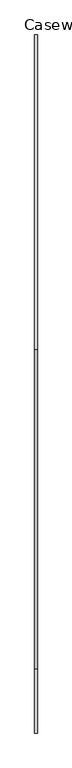
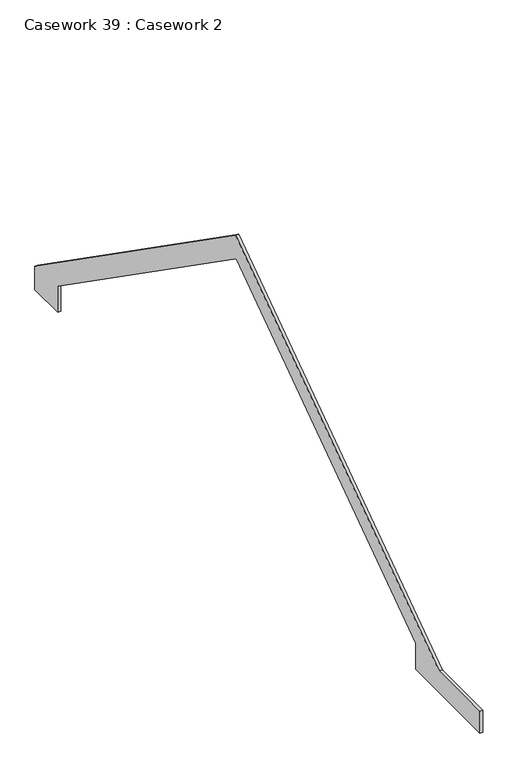
"""IFC4 building model written with IfcOpenShell, lengths in millimetres: furniture geometry, Casework 39 : Casework 2."""

from ifc_helpers import new_model, si_unit, frame, origin, place, context, project, spatial, polyline, outline, extrude, source, transform, mapped, element, save


def casework_39_casework_2_646cf92f(model_context):
    return source(origin(), model_context, "Body", "SweptSolid", [
        extrude(outline(polyline([(3156.9704867, 7937.1283557), (7125.8166964, 5158.1123216), (7125.8166964, 4875.3461918), (6675.8166964, 4875.3461918), (6675.8166964, 5190.0895255), (3151.1408768, 7658.0941041), (-400.040882, 5171.5298671), (-400.040882, 4860.0), (-1669.6462381, 4860.0), (-1669.6462381, 5121.8983063), (-863.5946969, 5121.8983063), (3156.9704867, 7937.1283557)])), frame((713.8336886, 0.0, 0.0), z_axis=(1.0, 0.0, 0.0), x_axis=(0.0, 1.0, 0.0)), (0.0, 0.0, 1.0), 33.2089356),
    ])


if __name__ == "__main__":
    model = new_model("IFC4")
    model_context = context("Model", 3, world=origin())
    ifc_project = project(units=[si_unit("LENGTHUNIT", "METRE", prefix="MILLI")], contexts=[model_context])
    site = spatial("IfcSite", under=ifc_project)
    building = spatial("IfcBuilding", under=site)
    placement = place(None, origin())
    casework_39_casework_2_shape = casework_39_casework_2_646cf92f(model_context)
    element("IfcFurniture", 1, ObjectType="Casework 39 : Casework 2", at=placement, inside=building, context=model_context, shape_type="MappedRepresentation", body=[
        mapped(casework_39_casework_2_shape, transform((0.0, 0.0, 0.0), x_axis=(1.0, 0.0, 0.0), y_axis=(0.0, 1.0, 0.0), z_axis=(0.0, 0.0, 1.0))),
    ])
    save(model, "model.ifc")

# Revit data of these elements
# Element 1 (IfcFurniture, "Casework 39 : Casework 2")
#   Materials on its faces: "Timber, Painted, White"
# Materials
#   "Timber, Painted, White": class "Wood", colour RGB 255 255 255, transparency 0, Comments = "Rendering appearance not upgraded ", Description = "Timber Barge Board, White Paint Finish", Cost = 0
